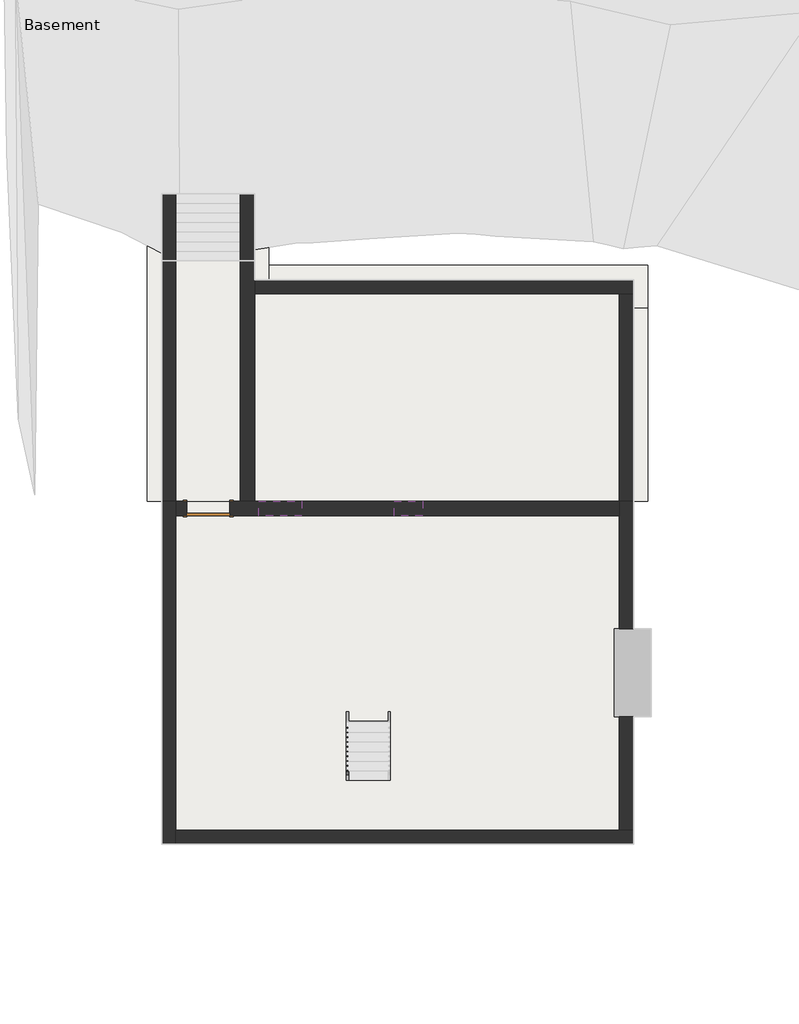
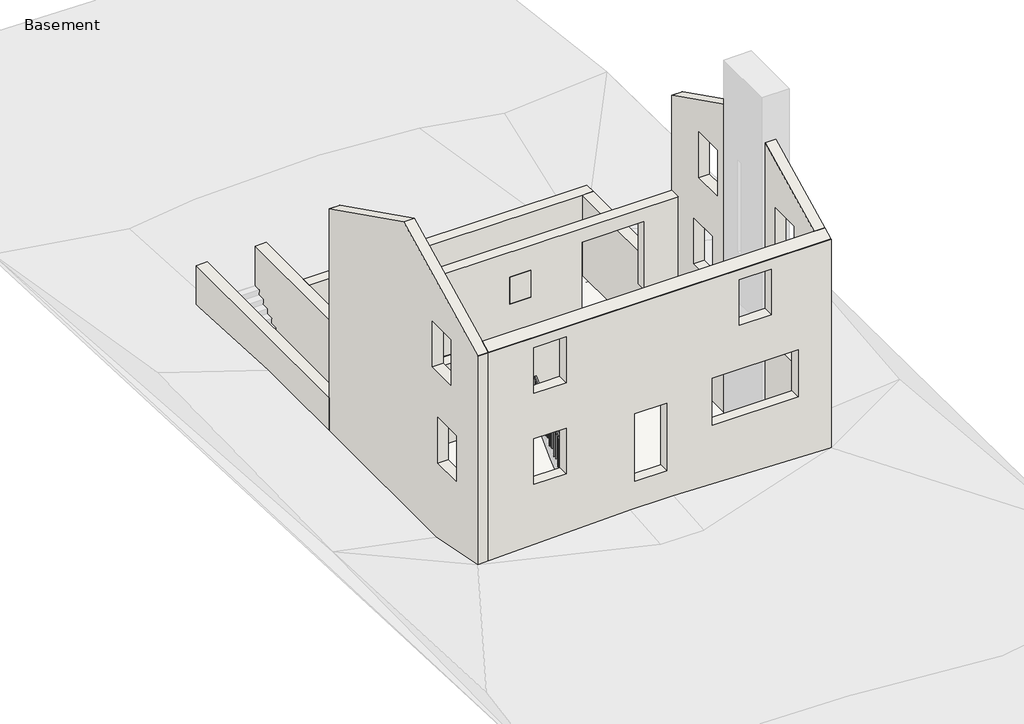
# One storey, part 1 of 2: 11 walls, 4 footings, 4 slabs, 1 door, 1 railing.
"""IFC4 building model written with IfcOpenShell, lengths in millimetres."""

import ifcopenshell
import ifcopenshell.guid

model = None  # the IFC model being written
_history = None  # IfcOwnerHistory: only IFC2X3 demands one
_inside = {}  # id of a spatial element -> (the spatial element, [elements in it])
_under = {}  # id of a project, library or spatial element -> (it, [spatial elements below it])
_declared = {}  # id of a project -> (the project, [libraries it declares])
_typed = {}  # id of a type object -> (the type object, [elements of that type])
_made_of = {}  # id of a material, layer set ... -> (it, [elements and type objects made of it])


def new_model(schema):
    """Start an empty IFC model of exactly this schema.

    Asked for "IFC4X3", IfcOpenShell would pick the latest addendum, in which some entities
    have other attributes; the version numbers below select the first issue.
    IFC2X3 requires an IfcOwnerHistory on every rooted entity: one is made here for all.
    """
    global model, _history
    if schema == "IFC4X3":
        model = ifcopenshell.file(schema_version=(4, 3, 0, 0))
    else:
        model = ifcopenshell.file(schema=schema)
    _inside.clear()
    _under.clear()
    _declared.clear()
    _typed.clear()
    _made_of.clear()
    _history = None
    if model.schema == "IFC2X3":
        org = make("IfcOrganization", Name="unknown")
        user = make(
            "IfcPersonAndOrganization",
            ThePerson=make("IfcPerson", FamilyName="unknown"),
            TheOrganization=org,
        )
        app = make(
            "IfcApplication",
            ApplicationDeveloper=org,
            Version="unknown",
            ApplicationFullName="unknown",
            ApplicationIdentifier="unknown",
        )
        _history = make(
            "IfcOwnerHistory",
            OwningUser=user,
            OwningApplication=app,
            ChangeAction="ADDED",
            CreationDate=0,
        )
    return model


def make(cls, **values):
    """One entity of the class cls with the attributes given. An attribute that is None is left unset."""
    return model.create_entity(
        cls, **{name: value for name, value in values.items() if value is not None}
    )


def rooted(cls, **values):
    """An entity with a GlobalId (a new one), such as an element, a storey or a relation."""
    return make(cls, GlobalId=ifcopenshell.guid.new(), OwnerHistory=_history, **values)


def si_unit(unit_type, name, prefix=None):
    """IfcSIUnit, for example si_unit("LENGTHUNIT", "METRE", prefix="MILLI")."""
    return make("IfcSIUnit", UnitType=unit_type, Prefix=prefix, Name=name)


def assignment(units):
    """IfcUnitAssignment: the units of a project."""
    return None if units is None else make("IfcUnitAssignment", Units=units)


def point(xyz):
    """IfcCartesianPoint."""
    return None if xyz is None else make("IfcCartesianPoint", Coordinates=xyz)


def direction(xyz):
    """IfcDirection."""
    return None if xyz is None else make("IfcDirection", DirectionRatios=xyz)


def frame(location, z_axis=None, x_axis=None):
    """IfcAxis2Placement3D, a coordinate frame: its origin and axes. An axis left out is left unset."""
    return make(
        "IfcAxis2Placement3D",
        Location=point(location),
        Axis=direction(z_axis),
        RefDirection=direction(x_axis),
    )


def origin():
    """The frame at (0, 0, 0) with its axes left unset."""
    return frame((0.0, 0.0, 0.0))


def origin_with_axes():
    """The frame at (0, 0, 0) with the z axis (0, 0, 1) and the x axis (1, 0, 0) written out."""
    return frame((0.0, 0.0, 0.0), z_axis=(0.0, 0.0, 1.0), x_axis=(1.0, 0.0, 0.0))


def place(relative_to, where):
    """IfcLocalPlacement: puts the frame where relative to a parent placement (None: the world)."""
    return make(
        "IfcLocalPlacement", PlacementRelTo=relative_to, RelativePlacement=where
    )


def context(
    kind, dimensions, precision=None, world=None, true_north=None, identifier=None
):
    """IfcGeometricRepresentationContext, for example the 3D "Model" context."""
    return make(
        "IfcGeometricRepresentationContext",
        ContextIdentifier=identifier,
        ContextType=kind,
        CoordinateSpaceDimension=dimensions,
        Precision=precision,
        WorldCoordinateSystem=world,
        TrueNorth=true_north,
    )


def project(units=None, contexts=None):
    """IfcProject with its units and contexts."""
    return rooted(
        "IfcProject",
        Name="project",
        RepresentationContexts=contexts,
        UnitsInContext=assignment(units),
    )


def spatial(cls, under=None, at=None, **own):
    """A site, building, storey or space (cls), placed at a placement, below another one or the project."""
    s = rooted(cls, ObjectPlacement=at, **own)
    if under is not None:
        _under.setdefault(under.id(), (under, []))[1].append(s)
    return s


def polyline(points):
    """IfcPolyline through the points."""
    return make("IfcPolyline", Points=[point(p) for p in points])


def outline(outer, holes=None, kind="AREA"):
    """IfcArbitraryClosedProfileDef: a profile drawn as a closed curve; with holes, ...WithVoids."""
    if holes is None:
        return make("IfcArbitraryClosedProfileDef", ProfileType=kind, OuterCurve=outer)
    return make(
        "IfcArbitraryProfileDefWithVoids",
        ProfileType=kind,
        OuterCurve=outer,
        InnerCurves=holes,
    )


def extrude(swept, where, along, depth):
    """IfcExtrudedAreaSolid: the profile swept, set in the frame where, extruded along a direction by depth."""
    return make(
        "IfcExtrudedAreaSolid",
        SweptArea=swept,
        Position=where,
        ExtrudedDirection=direction(along),
        Depth=depth,
    )


def faces_of(points, faces, orient=None, outer=None):
    """IfcFace entities. A face is a list of loops; a loop is a list of indices into points, from 0.

    orient and outer hold one flag for each loop. By default every Orientation is true, the
    first loop of a face is its IfcFaceOuterBound and the others are IfcFaceBound.
    """
    made = []
    for i, loops in enumerate(faces):
        bounds = []
        for j, loop in enumerate(loops):
            is_outer = j == 0 if outer is None else outer[i][j]
            bounds.append(
                make(
                    "IfcFaceOuterBound" if is_outer else "IfcFaceBound",
                    Bound=make("IfcPolyLoop", Polygon=[points[k] for k in loop]),
                    Orientation=True if orient is None else orient[i][j],
                )
            )
        made.append(make("IfcFace", Bounds=bounds))
    return made


def faceted_brep(points, faces, orient=None, outer=None, voids=None):
    """IfcFacetedBrep: a solid bounded by flat faces; with voids (closed shells), ...WithVoids."""
    shared = [point(p) for p in points]
    hull = make("IfcClosedShell", CfsFaces=faces_of(shared, faces, orient, outer))
    if voids is None:
        return make("IfcFacetedBrep", Outer=hull)
    return make(
        "IfcFacetedBrepWithVoids",
        Outer=hull,
        Voids=[
            make(cls, CfsFaces=faces_of(shared, fs, o, b)) for cls, fs, o, b in voids
        ],
    )


def shape(context_of_items, identifier, shape_type, items):
    """IfcShapeRepresentation: the items that make up one representation, for example the "Body"."""
    return make(
        "IfcShapeRepresentation",
        ContextOfItems=context_of_items,
        RepresentationIdentifier=identifier,
        RepresentationType=shape_type,
        Items=items,
    )


def source(mapping_origin, context_of_items, identifier, shape_type, items):
    """IfcRepresentationMap: a shape defined once, which mapped items show again and again."""
    return make(
        "IfcRepresentationMap",
        MappingOrigin=mapping_origin,
        MappedRepresentation=shape(context_of_items, identifier, shape_type, items),
    )


def transform(
    local_origin,
    x_axis=None,
    y_axis=None,
    z_axis=None,
    scale=None,
    scale2=None,
    scale3=None,
    uniform=True,
):
    """IfcCartesianTransformationOperator3D, or its non-uniform kind. x_axis, y_axis, z_axis: its Axis1, 2, 3."""
    if uniform:
        return make(
            "IfcCartesianTransformationOperator3D",
            Axis1=direction(x_axis),
            Axis2=direction(y_axis),
            LocalOrigin=point(local_origin),
            Scale=scale,
            Axis3=direction(z_axis),
        )
    return make(
        "IfcCartesianTransformationOperator3DnonUniform",
        Axis1=direction(x_axis),
        Axis2=direction(y_axis),
        LocalOrigin=point(local_origin),
        Scale=scale,
        Axis3=direction(z_axis),
        Scale2=scale2,
        Scale3=scale3,
    )


def mapped(mapping_source, mapping_target):
    """IfcMappedItem: shows the shape of a source again, moved by a transform."""
    return make(
        "IfcMappedItem", MappingSource=mapping_source, MappingTarget=mapping_target
    )


def made_of(thing, what):
    """Note that an element or type object is made of a material, layer set ...; save() writes the relation."""
    if what is not None:
        _made_of.setdefault(what.id(), (what, []))[1].append(thing)
    return thing


def element(
    cls,
    number,
    at=None,
    inside=None,
    cuts=None,
    type_object=None,
    material=None,
    context=None,
    identifier="Body",
    shape_type=None,
    held_by="IfcProductDefinitionShape",
    body=None,
    shapes=None,
    **own,
):
    """One element of the class cls, such as IfcWall. Its Tag is "e" and its number.

    at: its placement. inside: the storey or other place that contains it. cuts: it is an
    opening in that element (IfcRelVoidsElement). A single representation is given by context,
    identifier, shape_type and body (its items); several are given by shapes. held_by: the class
    of the entity that holds the representations. save() writes the other relations.
    """
    e = rooted(cls, Tag="e%d" % number, ObjectPlacement=at, **own)
    if body is not None:
        shapes = [shape(context, identifier, shape_type, body)]
    if shapes is not None:
        e.Representation = make(held_by, Representations=shapes)
    if inside is not None:
        _inside.setdefault(inside.id(), (inside, []))[1].append(e)
    if cuts is not None:
        rooted(
            "IfcRelVoidsElement", RelatingBuildingElement=cuts, RelatedOpeningElement=e
        )
    if type_object is not None:
        _typed.setdefault(type_object.id(), (type_object, []))[1].append(e)
    return made_of(e, material)


def aggregate(whole, parts):
    """IfcRelAggregates: a whole, such as a stair, and the parts it consists of."""
    return rooted("IfcRelAggregates", RelatingObject=whole, RelatedObjects=parts)


def save(model, path):
    """Write the relations noted so far, then the file.

    IfcRelAggregates (storeys below a building ...), IfcRelContainedInSpatialStructure (elements
    in a storey), IfcRelDefinesByType, IfcRelAssociatesMaterial and IfcRelDeclares: one each for
    every whole, place, type object, material and project.
    """
    for whole, parts in _under.values():
        aggregate(whole, parts)
    for where, things in _inside.values():
        rooted(
            "IfcRelContainedInSpatialStructure",
            RelatedElements=things,
            RelatingStructure=where,
        )
    for kind, things in _typed.values():
        rooted("IfcRelDefinesByType", RelatedObjects=things, RelatingType=kind)
    for what, things in _made_of.values():
        rooted("IfcRelAssociatesMaterial", RelatedObjects=things, RelatingMaterial=what)
    for by, libraries in _declared.values():
        rooted("IfcRelDeclares", RelatingContext=by, RelatedDefinitions=libraries)
    model.write(path)


def door_03272193(model_context):
    return source(origin(), model_context, "Body", "SweptSolid", [
        extrude(outline(polyline([(2209.8, -533.4), (0.0, -533.4), (0.0, -457.2), (2133.6, -457.2), (2133.6, 457.2), (0.0, 457.2), (0.0, 533.4), (2209.8, 533.4), (2209.8, -533.4)])), frame((0.0, 152.4, 0.0), z_axis=(0.0, 1.0, 0.0), x_axis=(0.0, 0.0, 1.0)), (0.0, 0.0, 1.0), 25.4),
        extrude(outline(polyline([(2209.8, 533.4), (2209.8, -533.4), (0.0, -533.4), (0.0, -457.2), (2133.6, -457.2), (2133.6, 457.2), (0.0, 457.2), (0.0, 533.4), (2209.8, 533.4)])), frame((0.0, -177.8, 0.0), z_axis=(0.0, 1.0, 0.0), x_axis=(0.0, 0.0, 1.0)), (0.0, 0.0, 1.0), 25.4),
        extrude(outline(polyline([(457.2, 101.6), (-457.2, 101.6), (-457.2, 152.4), (457.2, 152.4), (457.2, 101.6)])), origin_with_axes(), (0.0, 0.0, 1.0), 2133.6),
    ])


model = new_model("IFC4")

# Units and contexts
model_context = context("Model", 3, world=origin())
ifc_project = project(units=[si_unit("LENGTHUNIT", "METRE", prefix="MILLI")], contexts=[model_context])

# Site, building, storey
site = spatial("IfcSite", under=ifc_project)
building = spatial("IfcBuilding", under=site)
storey = spatial("IfcBuildingStorey", under=building, Name="Basement", Elevation=-2667.0)

# Door
placement = place(None, origin())
door_shape = door_03272193(model_context)
element("IfcDoor", 1, ObjectType="Single-Flush : 36\" x 84\"", at=placement, inside=storey, context=model_context, shape_type="MappedRepresentation", body=[
    mapped(door_shape, transform((-4998.5803068, 2999.6888758, -2667.0), x_axis=(-1.0, 0.0, 0.0), y_axis=(0.0, -1.0, 0.0), z_axis=(0.0, 0.0, 1.0))),
])

# Footings
element("IfcFooting", 2, ObjectType="Bearing Footing - 36\" x 12\"", at=placement, inside=storey, context=model_context, shape_type="SweptSolid", body=[
    extrude(outline(polyline([(-5379.5803068, 3152.0888758), (-6293.9803068, 3152.0888758), (-6293.9803068, 10010.0888758), (-5379.5803068, 10010.0888758), (-5379.5803068, 3152.0888758)])), frame((0.0, 0.0, -3073.4), z_axis=(0.0, 0.0, 1.0), x_axis=(1.0, 0.0, 0.0)), (0.0, 0.0, 1.0), 304.8),
])
element("IfcFooting", 3, ObjectType="Bearing Footing - 36\" x 12\"", at=placement, inside=storey, context=model_context, shape_type="Brep", body=[
    faceted_brep([(-3703.1803068, 7266.8888758, -2768.6), (3459.6196932, 7266.8888758, -2768.6), (4374.0196932, 7266.8888758, -2768.6), (4374.0196932, 8181.2888758, -2768.6), (-3703.1803068, 8181.2888758, -2768.6), (-3703.1803068, 8181.2888758, -3073.4), (4374.0196932, 8181.2888758, -3073.4), (-3703.1803068, 7266.8888758, -3073.4), (4374.0196932, 7266.8888758, -3073.4), (3459.6196932, 7266.8888758, -3073.4)], [[[0, 1, 2, 3, 4]], [[5, 4, 3, 6]], [[7, 5, 6, 8, 9]], [[0, 7, 9, 8, 2, 1]], [[0, 4, 5, 7]], [[3, 2, 8, 6]]]),
])
element("IfcFooting", 4, ObjectType="Bearing Footing - 36\" x 12\"", at=placement, inside=storey, context=model_context, shape_type="SweptSolid", body=[
    extrude(outline(polyline([(4374.0196932, 3152.0888758), (3459.6196932, 3152.0888758), (3459.6196932, 7266.8888758), (4374.0196932, 7266.8888758), (4374.0196932, 3152.0888758)])), frame((0.0, 0.0, -3073.4), z_axis=(0.0, 0.0, 1.0), x_axis=(1.0, 0.0, 0.0)), (0.0, 0.0, 1.0), 304.8),
])
element("IfcFooting", 5, ObjectType="Bearing Footing - 36\" x 12\"", at=placement, inside=storey, context=model_context, shape_type="Brep", body=[
    faceted_brep([(-3703.1803068, 3152.0888758, -2768.6), (-4617.5803068, 3152.0888758, -2768.6), (-4617.5803068, 3152.0888758, -3073.4), (-3703.1803068, 3152.0888758, -3073.4), (-4617.5803068, 10010.0888758, -2768.6), (-3703.1803068, 10010.0888758, -2768.6), (-3703.1803068, 10010.0888758, -3073.4), (-4617.5803068, 10010.0888758, -3073.4), (-3703.1803068, 7266.8888758, -2768.6), (-3703.1803068, 8181.2888758, -2768.6), (-3703.1803068, 8181.2888758, -3073.4), (-3703.1803068, 7266.8888758, -3073.4)], [[[0, 1, 2, 3]], [[4, 5, 6, 7]], [[0, 8, 9, 5, 4, 1]], [[2, 1, 4, 7]], [[3, 2, 7, 6, 10, 11]], [[0, 3, 11, 10, 6, 5, 9, 8]]]),
])

# Railing
element("IfcRailing", 6, ObjectType="Handrail - Rectangular", at=placement, inside=storey, context=model_context, shape_type="SweptSolid", body=[
    extrude(outline(polyline([(-2791.5111242, -1631.7331862), (-2791.5111242, -1562.1), (-149.9111242, 914.4), (-149.9111242, 844.7668138), (-2791.5111242, -1631.7331862)])), frame((-2052.1803068, 0.0, 0.0), z_axis=(1.0, 0.0, 0.0), x_axis=(0.0, 1.0, 0.0)), (0.0, 0.0, 1.0), 50.8),
    extrude(outline(polyline([(-241.9861242, 758.4465013), (-241.9861242, -190.5), (-261.0361242, -190.5), (-261.0361242, 740.5871263), (-241.9861242, 758.4465013)])), frame((-2036.3053068, 0.0, 0.0), z_axis=(1.0, 0.0, 0.0), x_axis=(0.0, 1.0, 0.0)), (0.0, 0.0, 1.0), 19.05),
    extrude(outline(polyline([(-343.5861242, 663.1965013), (-343.5861242, -190.5), (-362.6361242, -190.5), (-362.6361242, 645.3371263), (-343.5861242, 663.1965013)])), frame((-2036.3053068, 0.0, 0.0), z_axis=(1.0, 0.0, 0.0), x_axis=(0.0, 1.0, 0.0)), (0.0, 0.0, 1.0), 19.05),
    extrude(outline(polyline([(-445.1861242, 567.9465013), (-445.1861242, -381.0), (-464.2361242, -381.0), (-464.2361242, 550.0871263), (-445.1861242, 567.9465013)])), frame((-2036.3053068, 0.0, 0.0), z_axis=(1.0, 0.0, 0.0), x_axis=(0.0, 1.0, 0.0)), (0.0, 0.0, 1.0), 19.05),
    extrude(outline(polyline([(-546.7861242, 472.6965013), (-546.7861242, -381.0), (-565.8361242, -381.0), (-565.8361242, 454.8371263), (-546.7861242, 472.6965013)])), frame((-2036.3053068, 0.0, 0.0), z_axis=(1.0, 0.0, 0.0), x_axis=(0.0, 1.0, 0.0)), (0.0, 0.0, 1.0), 19.05),
    extrude(outline(polyline([(-648.3861242, 377.4465013), (-648.3861242, -571.5), (-667.4361242, -571.5), (-667.4361242, 359.5871263), (-648.3861242, 377.4465013)])), frame((-2036.3053068, 0.0, 0.0), z_axis=(1.0, 0.0, 0.0), x_axis=(0.0, 1.0, 0.0)), (0.0, 0.0, 1.0), 19.05),
    extrude(outline(polyline([(-749.9861242, 282.1965013), (-749.9861242, -571.5), (-769.0361242, -571.5), (-769.0361242, 264.3371263), (-749.9861242, 282.1965013)])), frame((-2036.3053068, 0.0, 0.0), z_axis=(1.0, 0.0, 0.0), x_axis=(0.0, 1.0, 0.0)), (0.0, 0.0, 1.0), 19.05),
    extrude(outline(polyline([(-851.5861242, 186.9465013), (-851.5861242, -762.0), (-870.6361242, -762.0), (-870.6361242, 169.0871263), (-851.5861242, 186.9465013)])), frame((-2036.3053068, 0.0, 0.0), z_axis=(1.0, 0.0, 0.0), x_axis=(0.0, 1.0, 0.0)), (0.0, 0.0, 1.0), 19.05),
    extrude(outline(polyline([(-953.1861242, 91.6965013), (-953.1861242, -762.0), (-972.2361242, -762.0), (-972.2361242, 73.8371263), (-953.1861242, 91.6965013)])), frame((-2036.3053068, 0.0, 0.0), z_axis=(1.0, 0.0, 0.0), x_axis=(0.0, 1.0, 0.0)), (0.0, 0.0, 1.0), 19.05),
    extrude(outline(polyline([(-1054.7861242, -3.5534987), (-1054.7861242, -952.5), (-1073.8361242, -952.5), (-1073.8361242, -21.4128737), (-1054.7861242, -3.5534987)])), frame((-2036.3053068, 0.0, 0.0), z_axis=(1.0, 0.0, 0.0), x_axis=(0.0, 1.0, 0.0)), (0.0, 0.0, 1.0), 19.05),
    extrude(outline(polyline([(-1156.3861242, -98.8034987), (-1156.3861242, -952.5), (-1175.4361242, -952.5), (-1175.4361242, -116.6628737), (-1156.3861242, -98.8034987)])), frame((-2036.3053068, 0.0, 0.0), z_axis=(1.0, 0.0, 0.0), x_axis=(0.0, 1.0, 0.0)), (0.0, 0.0, 1.0), 19.05),
    extrude(outline(polyline([(-1257.9861242, -194.0534987), (-1257.9861242, -1143.0), (-1277.0361242, -1143.0), (-1277.0361242, -211.9128737), (-1257.9861242, -194.0534987)])), frame((-2036.3053068, 0.0, 0.0), z_axis=(1.0, 0.0, 0.0), x_axis=(0.0, 1.0, 0.0)), (0.0, 0.0, 1.0), 19.05),
    extrude(outline(polyline([(-1359.5861242, -289.3034987), (-1359.5861242, -1143.0), (-1378.6361242, -1143.0), (-1378.6361242, -307.1628737), (-1359.5861242, -289.3034987)])), frame((-2036.3053068, 0.0, 0.0), z_axis=(1.0, 0.0, 0.0), x_axis=(0.0, 1.0, 0.0)), (0.0, 0.0, 1.0), 19.05),
    extrude(outline(polyline([(-1461.1861242, -384.5534987), (-1461.1861242, -1333.5), (-1480.2361242, -1333.5), (-1480.2361242, -402.4128737), (-1461.1861242, -384.5534987)])), frame((-2036.3053068, 0.0, 0.0), z_axis=(1.0, 0.0, 0.0), x_axis=(0.0, 1.0, 0.0)), (0.0, 0.0, 1.0), 19.05),
    extrude(outline(polyline([(-1562.7861242, -479.8034987), (-1562.7861242, -1333.5), (-1581.8361242, -1333.5), (-1581.8361242, -497.6628737), (-1562.7861242, -479.8034987)])), frame((-2036.3053068, 0.0, 0.0), z_axis=(1.0, 0.0, 0.0), x_axis=(0.0, 1.0, 0.0)), (0.0, 0.0, 1.0), 19.05),
    extrude(outline(polyline([(-1664.3861242, -575.0534987), (-1664.3861242, -1524.0), (-1683.4361242, -1524.0), (-1683.4361242, -592.9128737), (-1664.3861242, -575.0534987)])), frame((-2036.3053068, 0.0, 0.0), z_axis=(1.0, 0.0, 0.0), x_axis=(0.0, 1.0, 0.0)), (0.0, 0.0, 1.0), 19.05),
    extrude(outline(polyline([(-1765.9861242, -670.3034987), (-1765.9861242, -1524.0), (-1785.0361242, -1524.0), (-1785.0361242, -688.1628737), (-1765.9861242, -670.3034987)])), frame((-2036.3053068, 0.0, 0.0), z_axis=(1.0, 0.0, 0.0), x_axis=(0.0, 1.0, 0.0)), (0.0, 0.0, 1.0), 19.05),
    extrude(outline(polyline([(-1867.5861242, -765.5534987), (-1867.5861242, -1714.5), (-1886.6361242, -1714.5), (-1886.6361242, -783.4128737), (-1867.5861242, -765.5534987)])), frame((-2036.3053068, 0.0, 0.0), z_axis=(1.0, 0.0, 0.0), x_axis=(0.0, 1.0, 0.0)), (0.0, 0.0, 1.0), 19.05),
    extrude(outline(polyline([(-1969.1861242, -860.8034987), (-1969.1861242, -1714.5), (-1988.2361242, -1714.5), (-1988.2361242, -878.6628737), (-1969.1861242, -860.8034987)])), frame((-2036.3053068, 0.0, 0.0), z_axis=(1.0, 0.0, 0.0), x_axis=(0.0, 1.0, 0.0)), (0.0, 0.0, 1.0), 19.05),
    extrude(outline(polyline([(-2070.7861242, -956.0534987), (-2070.7861242, -1905.0), (-2089.8361242, -1905.0), (-2089.8361242, -973.9128737), (-2070.7861242, -956.0534987)])), frame((-2036.3053068, 0.0, 0.0), z_axis=(1.0, 0.0, 0.0), x_axis=(0.0, 1.0, 0.0)), (0.0, 0.0, 1.0), 19.05),
    extrude(outline(polyline([(-2172.3861242, -1051.3034987), (-2172.3861242, -1905.0), (-2191.4361242, -1905.0), (-2191.4361242, -1069.1628737), (-2172.3861242, -1051.3034987)])), frame((-2036.3053068, 0.0, 0.0), z_axis=(1.0, 0.0, 0.0), x_axis=(0.0, 1.0, 0.0)), (0.0, 0.0, 1.0), 19.05),
    extrude(outline(polyline([(-2273.9861242, -1146.5534987), (-2273.9861242, -2095.5), (-2293.0361242, -2095.5), (-2293.0361242, -1164.4128737), (-2273.9861242, -1146.5534987)])), frame((-2036.3053068, 0.0, 0.0), z_axis=(1.0, 0.0, 0.0), x_axis=(0.0, 1.0, 0.0)), (0.0, 0.0, 1.0), 19.05),
    extrude(outline(polyline([(-2375.5861242, -1241.8034987), (-2375.5861242, -2095.5), (-2394.6361242, -2095.5), (-2394.6361242, -1259.6628737), (-2375.5861242, -1241.8034987)])), frame((-2036.3053068, 0.0, 0.0), z_axis=(1.0, 0.0, 0.0), x_axis=(0.0, 1.0, 0.0)), (0.0, 0.0, 1.0), 19.05),
    extrude(outline(polyline([(-2477.1861242, -1337.0534987), (-2477.1861242, -2286.0), (-2496.2361242, -2286.0), (-2496.2361242, -1354.9128737), (-2477.1861242, -1337.0534987)])), frame((-2036.3053068, 0.0, 0.0), z_axis=(1.0, 0.0, 0.0), x_axis=(0.0, 1.0, 0.0)), (0.0, 0.0, 1.0), 19.05),
    extrude(outline(polyline([(-2578.7861242, -1432.3034987), (-2578.7861242, -2286.0), (-2597.8361242, -2286.0), (-2597.8361242, -1450.1628737), (-2578.7861242, -1432.3034987)])), frame((-2036.3053068, 0.0, 0.0), z_axis=(1.0, 0.0, 0.0), x_axis=(0.0, 1.0, 0.0)), (0.0, 0.0, 1.0), 19.05),
    extrude(outline(polyline([(-2680.3861242, -1527.5534987), (-2680.3861242, -2476.5), (-2699.4361242, -2476.5), (-2699.4361242, -1545.4128737), (-2680.3861242, -1527.5534987)])), frame((-2036.3053068, 0.0, 0.0), z_axis=(1.0, 0.0, 0.0), x_axis=(0.0, 1.0, 0.0)), (0.0, 0.0, 1.0), 19.05),
    extrude(outline(polyline([(-149.9111242, 844.7668138), (-149.9111242, -190.5), (-168.9611242, -190.5), (-168.9611242, 826.9074388), (-149.9111242, 844.7668138)])), frame((-2036.3053068, 0.0, 0.0), z_axis=(1.0, 0.0, 0.0), x_axis=(0.0, 1.0, 0.0)), (0.0, 0.0, 1.0), 19.05),
    extrude(outline(polyline([(-2772.4611242, -1613.8738112), (-2772.4611242, -2476.5), (-2791.5111242, -2476.5), (-2791.5111242, -1631.7331862), (-2772.4611242, -1613.8738112)])), frame((-2036.3053068, 0.0, 0.0), z_axis=(1.0, 0.0, 0.0), x_axis=(0.0, 1.0, 0.0)), (0.0, 0.0, 1.0), 19.05),
])

# Slabs
element("IfcSlab", 7, ObjectType="4\" Concrete", at=placement, inside=storey, context=model_context, shape_type="SweptSolid", body=[
    extrude(outline(polyline([(-5684.3803068, 8384.4888758), (-4312.7803068, 8384.4888758), (-4312.7803068, 3152.0888758), (-5684.3803068, 3152.0888758), (-5684.3803068, 8384.4888758)])), frame((0.0, 0.0, -2768.6), z_axis=(0.0, 0.0, 1.0), x_axis=(1.0, 0.0, 0.0)), (0.0, 0.0, 1.0), 101.6),
])
element("IfcSlab", 8, ObjectType="Pad 1", at=placement, inside=storey, context=model_context, shape_type="SweptSolid", body=[
    extrude(outline(polyline([(4069.2196932, 434.2888758), (4450.2196932, 434.2888758), (4450.2196932, -1445.3111242), (4069.2196932, -1445.3111242), (4069.2196932, -4163.1111242), (-5989.1803068, -4163.1111242), (-5989.1803068, 3152.0888758), (4069.2196932, 3152.0888758), (4069.2196932, 434.2888758)])), frame((0.0, 0.0, -3073.4), z_axis=(0.0, 0.0, 1.0), x_axis=(1.0, 0.0, 0.0)), (0.0, 0.0, 1.0), 304.8),
])
element("IfcSlab", 9, ObjectType="Pad 1", at=placement, inside=storey, context=model_context, shape_type="SweptSolid", body=[
    extrude(outline(polyline([(-5989.1803068, 8275.4102719), (-4007.9803068, 8275.4102719), (-4007.9803068, 7876.4888758), (4069.2196932, 7876.4888758), (4069.2196932, 3152.0888758), (-5989.1803068, 3152.0888758), (-5989.1803068, 8275.4102719)])), frame((0.0, 0.0, -3073.4), z_axis=(0.0, 0.0, 1.0), x_axis=(1.0, 0.0, 0.0)), (0.0, 0.0, 1.0), 304.8),
])
element("IfcSlab", 10, ObjectType="Under Stairs", at=placement, inside=storey, context=model_context, shape_type="SweptSolid", body=[
    extrude(outline(polyline([(9705.2888758, -1653.200634), (8275.4102719, -2776.6756068), (8275.4102719, -2768.6), (9705.2888758, -1645.1250272), (9705.2888758, -1653.200634)])), frame((-5989.1803068, 0.0, 0.0), z_axis=(1.0, 0.0, 0.0), x_axis=(0.0, 1.0, 0.0)), (0.0, 0.0, 1.0), 1981.2),
])

# Walls
element("IfcWall", 11, ObjectType="Foundation - 12\" Concrete", at=placement, inside=storey, context=model_context, shape_type="Brep", body=[
    faceted_brep([(-5684.3803068, 3152.0888758, -2768.6), (-5684.3803068, 8384.4888758, -2768.6), (-5684.3803068, 9705.2888758, -2768.6), (-5684.3803068, 9705.2888758, -349.25), (-5684.3803068, 3152.0888758, -349.25), (-5684.3803068, 3152.0888758, -2667.0), (-5989.1803068, 3152.0888758, -2768.6), (-5989.1803068, 3152.0888758, -349.25), (-5989.1803068, 9705.2888758, -349.25), (-5989.1803068, 9705.2888758, -2768.6)], [[[0, 1, 2, 3, 4, 5]], [[6, 7, 8, 9]], [[2, 1, 0, 6, 9]], [[3, 2, 9, 8]], [[4, 3, 8, 7]], [[0, 5, 4, 7, 6]]]),
])
element("IfcWall", 12, ObjectType="Foundation - 12\" Concrete", at=placement, inside=storey, context=model_context, shape_type="Brep", body=[
    faceted_brep([(-4007.9803068, 7571.6888758, -2768.6), (3764.4196932, 7571.6888758, -2768.6), (4069.2196932, 7571.6888758, -2768.6), (4069.2196932, 7571.6888758, -349.25), (3764.4196932, 7571.6888758, -349.25), (-4007.9803068, 7571.6888758, -349.25), (-4007.9803068, 7876.4888758, -2768.6), (-4007.9803068, 7876.4888758, -349.25), (4069.2196932, 7876.4888758, -349.25), (4069.2196932, 7876.4888758, -2768.6)], [[[0, 1, 2, 3, 4, 5]], [[6, 7, 8, 9]], [[2, 1, 0, 6, 9]], [[5, 4, 3, 8, 7]], [[3, 2, 9, 8]], [[0, 5, 7, 6]]]),
])
element("IfcWall", 13, ObjectType="Foundation - 12\" Concrete", at=placement, inside=storey, context=model_context, shape_type="Brep", body=[
    faceted_brep([(3764.4196932, 7571.6888758, -2768.6), (3764.4196932, 3152.0888758, -2768.6), (3764.4196932, 3152.0888758, -349.25), (3764.4196932, 7571.6888758, -349.25), (4069.2196932, 7571.6888758, -2768.6), (4069.2196932, 7571.6888758, -349.25), (4069.2196932, 7524.0638758, -349.25), (4069.2196932, 3152.0888758, -349.25), (4069.2196932, 3152.0888758, -2768.6)], [[[0, 1, 2, 3]], [[4, 5, 6, 7, 8]], [[1, 0, 4, 8]], [[3, 2, 7, 6, 5]], [[2, 1, 8, 7]], [[0, 3, 5, 4]]]),
])
element("IfcWall", 14, ObjectType="Foundation - 12\" Concrete", at=placement, inside=storey, context=model_context, shape_type="Brep", body=[
    faceted_brep([(-4007.9803068, 3152.0888758, -2768.6), (-4007.9803068, 7571.6888758, -2768.6), (-4007.9803068, 7876.4888758, -2768.6), (-4007.9803068, 9705.2888758, -2768.6), (-4007.9803068, 9705.2888758, -349.25), (-4007.9803068, 7876.4888758, -349.25), (-4007.9803068, 7571.6888758, -349.25), (-4007.9803068, 3152.0888758, -349.25), (-4312.7803068, 3152.0888758, -2768.6), (-4312.7803068, 3152.0888758, -2667.0), (-4312.7803068, 3152.0888758, -349.25), (-4312.7803068, 9705.2888758, -349.25), (-4312.7803068, 9705.2888758, -2768.6), (-4312.7803068, 8384.4888758, -2768.6)], [[[0, 1, 2, 3, 4, 5, 6, 7]], [[8, 9, 10, 11, 12, 13]], [[3, 2, 1, 0, 8, 13, 12]], [[4, 3, 12, 11]], [[7, 6, 5, 4, 11, 10]], [[0, 7, 10, 9, 8]]]),
])
element("IfcWall", 15, ObjectType="Generic - 12\"", at=placement, inside=storey, context=model_context, shape_type="Brep", body=[
    faceted_brep([(1021.2196932, 2847.2888758, 0.0), (1021.2196932, 2847.2888758, 2057.4), (2799.2196932, 2847.2888758, 2057.4), (2799.2196932, 2847.2888758, 0.0), (3764.4196932, 2847.2888758, 0.0), (3764.4196932, 2847.2888758, 2470.15), (-5684.3803068, 2847.2888758, 2470.15), (-5684.3803068, 2847.2888758, 0.0), (-5023.9803068, 2847.2888758, 0.0), (-5023.9803068, 2847.2888758, 2032.0), (-4160.3803068, 2847.2888758, 2032.0), (-4160.3803068, 2847.2888758, 0.0), (-1518.7803068, 2847.2888758, 0.0), (-1391.7803068, 2847.2888758, 0.0), (-70.9803068, 2847.2888758, 0.0), (56.0196932, 2847.2888758, 0.0), (-3919.0803068, 2847.2888758, 914.4), (-3919.0803068, 2847.2888758, 1727.2), (-3004.6803068, 2847.2888758, 1727.2), (-3004.6803068, 2847.2888758, 914.4), (-1036.1803068, 2847.2888758, 914.4), (-1036.1803068, 2847.2888758, 1727.2), (-426.5803068, 2847.2888758, 1727.2), (-426.5803068, 2847.2888758, 914.4), (1021.2196932, 3152.0888758, 2057.4), (1021.2196932, 3152.0888758, 0.0), (-4160.3803068, 3152.0888758, 0.0), (-4160.3803068, 3152.0888758, 2032.0), (-5023.9803068, 3152.0888758, 2032.0), (-5023.9803068, 3152.0888758, 0.0), (-5684.3803068, 3152.0888758, 0.0), (-5684.3803068, 3152.0888758, 2470.15), (3764.4196932, 3152.0888758, 2470.15), (3764.4196932, 3152.0888758, 0.0), (2799.2196932, 3152.0888758, 0.0), (2799.2196932, 3152.0888758, 2057.4), (-3919.0803068, 3152.0888758, 1727.2), (-3919.0803068, 3152.0888758, 914.4), (-3004.6803068, 3152.0888758, 914.4), (-3004.6803068, 3152.0888758, 1727.2), (-1036.1803068, 3152.0888758, 1727.2), (-1036.1803068, 3152.0888758, 914.4), (-426.5803068, 3152.0888758, 914.4), (-426.5803068, 3152.0888758, 1727.2)], [[[0, 1, 2, 3, 4, 5, 6, 7, 8, 9, 10, 11, 12, 13, 14, 15], [16, 17, 18, 19], [20, 21, 22, 23]], [[24, 25, 26, 27, 28, 29, 30, 31, 32, 33, 34, 35], [36, 37, 38, 39], [40, 41, 42, 43]], [[24, 1, 0, 25]], [[1, 24, 35, 2]], [[2, 35, 34, 3]], [[9, 8, 29, 28]], [[10, 9, 28, 27]], [[11, 10, 27, 26]], [[8, 7, 30, 29]], [[4, 3, 34, 33]], [[0, 15, 14, 13, 12, 11, 26, 25]], [[6, 5, 32, 31]], [[4, 33, 32, 5]], [[36, 17, 16, 37]], [[37, 16, 19, 38]], [[38, 19, 18, 39]], [[17, 36, 39, 18]], [[40, 21, 20, 41]], [[41, 20, 23, 42]], [[42, 23, 22, 43]], [[21, 40, 43, 22]], [[30, 7, 6, 31]]]),
    faceted_brep([(3764.4196932, 2847.2888758, -273.05), (-5684.3803068, 2847.2888758, -273.05), (-5684.3803068, 2847.2888758, -2667.0), (-5455.7803068, 2847.2888758, -2667.0), (-5455.7803068, 2847.2888758, -533.4), (-4541.3803068, 2847.2888758, -533.4), (-4541.3803068, 2847.2888758, -2667.0), (3764.4196932, 2847.2888758, -2667.0), (-5684.3803068, 3152.0888758, -273.05), (3764.4196932, 3152.0888758, -273.05), (3764.4196932, 3152.0888758, -2667.0), (-4541.3803068, 3152.0888758, -2667.0), (-4541.3803068, 3152.0888758, -533.4), (-5455.7803068, 3152.0888758, -533.4), (-5455.7803068, 3152.0888758, -2667.0), (-5684.3803068, 3152.0888758, -2667.0)], [[[0, 1, 2, 3, 4, 5, 6, 7]], [[8, 9, 10, 11, 12, 13, 14, 15]], [[10, 7, 6, 11]], [[3, 2, 15, 14]], [[1, 0, 9, 8]], [[7, 10, 9, 0]], [[13, 4, 3, 14]], [[4, 13, 12, 5]], [[5, 12, 11, 6]], [[15, 2, 1, 8]]]),
])
element("IfcWall", 16, ObjectType="Generic - 12\"", at=placement, inside=storey, context=model_context, shape_type="Brep", body=[
    faceted_brep([(-5684.3803068, -4163.1111242, -2667.0), (-5684.3803068, -3858.3111242, -2667.0), (-5684.3803068, 2847.2888758, -2667.0), (-5684.3803068, 3152.0888758, -2667.0), (-5684.3803068, 3152.0888758, -273.05), (-5684.3803068, 3152.0888758, 0.0), (-5684.3803068, 3152.0888758, 2470.15), (-5684.3803068, 3152.0888758, 5336.1342644), (-5684.3803068, 3147.820347, 5336.1342644), (-5684.3803068, -505.5111242, 7162.8), (-5684.3803068, -3858.3111242, 5486.4), (-5684.3803068, -4158.8425953, 5336.1342644), (-5684.3803068, -4163.1111242, 5336.1342644), (-5684.3803068, -3096.3111242, 914.4), (-5684.3803068, -3096.3111242, 2286.0), (-5684.3803068, -2181.9111242, 2286.0), (-5684.3803068, -2181.9111242, 914.4), (-5684.3803068, -2842.3111242, 3657.6), (-5684.3803068, -2842.3111242, 5029.2), (-5684.3803068, -1927.9111242, 5029.2), (-5684.3803068, -1927.9111242, 3657.6), (-5989.1803068, 3152.0888758, -2667.0), (-5989.1803068, -4163.1111242, -2667.0), (-5989.1803068, -4163.1111242, 5336.1342644), (-5989.1803068, -4158.8425953, 5336.1342644), (-5989.1803068, -505.5111242, 7162.8), (-5989.1803068, 3147.820347, 5336.1342644), (-5989.1803068, 3152.0888758, 5336.1342644), (-5989.1803068, -3096.3111242, 2286.0), (-5989.1803068, -3096.3111242, 914.4), (-5989.1803068, -2181.9111242, 914.4), (-5989.1803068, -2181.9111242, 2286.0), (-5989.1803068, -2842.3111242, 5029.2), (-5989.1803068, -2842.3111242, 3657.6), (-5989.1803068, -1927.9111242, 3657.6), (-5989.1803068, -1927.9111242, 5029.2)], [[[0, 1, 2, 3, 4, 5, 6, 7, 8, 9, 10, 11, 12], [13, 14, 15, 16], [17, 18, 19, 20]], [[21, 22, 23, 24, 25, 26, 27], [28, 29, 30, 31], [32, 33, 34, 35]], [[3, 2, 1, 0, 22, 21]], [[0, 12, 23, 22]], [[29, 28, 14, 13]], [[30, 29, 13, 16]], [[31, 30, 16, 15]], [[28, 31, 15, 14]], [[32, 18, 17, 33]], [[33, 17, 20, 34]], [[34, 20, 19, 35]], [[18, 32, 35, 19]], [[23, 12, 11, 24]], [[25, 24, 11, 10, 9]], [[9, 8, 26, 25]], [[8, 7, 27, 26]], [[3, 21, 27, 7, 6, 5, 4]]]),
])
element("IfcWall", 17, ObjectType="Generic - 12\"", at=placement, inside=storey, context=model_context, shape_type="Brep", body=[
    faceted_brep([(4069.2196932, -3858.3111242, -2667.0), (3764.4196932, -3858.3111242, -2667.0), (-5684.3803068, -3858.3111242, -2667.0), (-5684.3803068, -3858.3111242, 5486.4), (3764.4196932, -3858.3111242, 5486.4), (4069.2196932, -3858.3111242, 5486.4), (-1518.7803068, -3858.3111242, 0.0), (-604.3803068, -3858.3111242, 0.0), (-604.3803068, -3858.3111242, 2032.0), (-1518.7803068, -3858.3111242, 2032.0), (-3474.5803068, -3858.3111242, 914.4), (-3474.5803068, -3858.3111242, 2286.0), (-4388.9803068, -3858.3111242, 2286.0), (-4388.9803068, -3858.3111242, 914.4), (2367.4196932, -3858.3111242, 3657.6), (2367.4196932, -3858.3111242, 5029.2), (1453.0196932, -3858.3111242, 5029.2), (1453.0196932, -3858.3111242, 3657.6), (-3474.5803068, -3858.3111242, 3657.6), (-3474.5803068, -3858.3111242, 5029.2), (-4388.9803068, -3858.3111242, 5029.2), (-4388.9803068, -3858.3111242, 3657.6), (3129.4196932, -3858.3111242, 2336.8), (691.0196932, -3858.3111242, 2336.8), (691.0196932, -3858.3111242, 914.4), (3129.4196932, -3858.3111242, 914.4), (-5684.3803068, -4163.1111242, -2667.0), (4069.2196932, -4163.1111242, -2667.0), (4069.2196932, -4163.1111242, 5336.1342644), (-5684.3803068, -4163.1111242, 5336.1342644), (-604.3803068, -4163.1111242, 0.0), (-1518.7803068, -4163.1111242, 0.0), (-1518.7803068, -4163.1111242, 2032.0), (-604.3803068, -4163.1111242, 2032.0), (-3474.5803068, -4163.1111242, 2286.0), (-3474.5803068, -4163.1111242, 914.4), (-4388.9803068, -4163.1111242, 914.4), (-4388.9803068, -4163.1111242, 2286.0), (2367.4196932, -4163.1111242, 5029.2), (2367.4196932, -4163.1111242, 3657.6), (1453.0196932, -4163.1111242, 3657.6), (1453.0196932, -4163.1111242, 5029.2), (-3474.5803068, -4163.1111242, 5029.2), (-3474.5803068, -4163.1111242, 3657.6), (-4388.9803068, -4163.1111242, 3657.6), (-4388.9803068, -4163.1111242, 5029.2), (3129.4196932, -4163.1111242, 914.4), (691.0196932, -4163.1111242, 914.4), (691.0196932, -4163.1111242, 2336.8), (3129.4196932, -4163.1111242, 2336.8), (4069.2196932, -4158.8425953, 5336.1342644), (-5684.3803068, -4158.8425953, 5336.1342644)], [[[0, 1, 2, 3, 4, 5], [6, 7, 8, 9], [10, 11, 12, 13], [14, 15, 16, 17], [18, 19, 20, 21], [22, 23, 24, 25]], [[26, 27, 28, 29], [30, 31, 32, 33], [34, 35, 36, 37], [38, 39, 40, 41], [42, 43, 44, 45], [46, 47, 48, 49]], [[2, 1, 0, 27, 26]], [[0, 5, 50, 28, 27]], [[3, 2, 26, 29, 51]], [[31, 30, 7, 6]], [[32, 31, 6, 9]], [[33, 32, 9, 8]], [[30, 33, 8, 7]], [[35, 34, 11, 10]], [[36, 35, 10, 13]], [[37, 36, 13, 12]], [[34, 37, 12, 11]], [[24, 47, 46, 25]], [[48, 23, 22, 49]], [[23, 48, 47, 24]], [[25, 46, 49, 22]], [[15, 14, 39, 38]], [[14, 17, 40, 39]], [[17, 16, 41, 40]], [[16, 15, 38, 41]], [[19, 18, 43, 42]], [[18, 21, 44, 43]], [[21, 20, 45, 44]], [[20, 19, 42, 45]], [[5, 4, 3, 51, 50]], [[29, 28, 50, 51]]]),
])
element("IfcWall", 18, ObjectType="Generic - 12\"", at=placement, inside=storey, context=model_context, shape_type="Brep", body=[
    faceted_brep([(3764.4196932, 3152.0888758, -2667.0), (3764.4196932, 2847.2888758, -2667.0), (3764.4196932, 434.2888758, -2667.0), (3764.4196932, 434.2888758, 6692.9), (3764.4196932, 2847.2888758, 5486.4), (3764.4196932, 3147.820347, 5336.1342644), (3764.4196932, 3152.0888758, 5336.1342644), (3764.4196932, 3152.0888758, 2743.2), (3764.4196932, 3152.0888758, 2470.15), (3764.4196932, 3152.0888758, 0.0), (3764.4196932, 3152.0888758, -273.05), (3764.4196932, 2085.2888758, 2286.0), (3764.4196932, 1170.8888758, 2286.0), (3764.4196932, 1170.8888758, 914.4), (3764.4196932, 2085.2888758, 914.4), (3764.4196932, 1831.2888758, 3657.6), (3764.4196932, 1831.2888758, 5029.2), (3764.4196932, 916.8888758, 5029.2), (3764.4196932, 916.8888758, 3657.6), (4069.2196932, 434.2888758, -2667.0), (4069.2196932, 3152.0888758, -2667.0), (4069.2196932, 3152.0888758, 5336.1342644), (4069.2196932, 3147.820347, 5336.1342644), (4069.2196932, 434.2888758, 6692.9), (4069.2196932, 2085.2888758, 2286.0), (4069.2196932, 2085.2888758, 914.4), (4069.2196932, 1170.8888758, 914.4), (4069.2196932, 1170.8888758, 2286.0), (4069.2196932, 1831.2888758, 5029.2), (4069.2196932, 1831.2888758, 3657.6), (4069.2196932, 916.8888758, 3657.6), (4069.2196932, 916.8888758, 5029.2)], [[[0, 1, 2, 3, 4, 5, 6, 7, 8, 9, 10], [11, 12, 13, 14], [15, 16, 17, 18]], [[19, 20, 21, 22, 23], [24, 25, 26, 27], [28, 29, 30, 31]], [[2, 1, 0, 20, 19]], [[3, 2, 19, 23]], [[25, 24, 11, 14]], [[26, 25, 14, 13]], [[27, 26, 13, 12]], [[24, 27, 12, 11]], [[28, 16, 15, 29]], [[29, 15, 18, 30]], [[30, 18, 17, 31]], [[16, 28, 31, 17]], [[21, 6, 5, 22]], [[3, 23, 22, 5, 4]], [[6, 21, 20, 0, 10, 9, 8, 7]]]),
])
element("IfcWall", 19, ObjectType="Generic - 12\"", at=placement, inside=storey, context=model_context, shape_type="SweptSolid", body=[
    extrude(outline(polyline([(-1445.3111242, -2667.0), (-3858.3111242, -2667.0), (-3858.3111242, 5486.4), (-1445.3111242, 6692.9), (-1445.3111242, -2667.0)]), holes=[polyline([(-2181.9111242, 2286.0), (-3096.3111242, 2286.0), (-3096.3111242, 914.4), (-2181.9111242, 914.4), (-2181.9111242, 2286.0)]), polyline([(-1927.9111242, 3657.6), (-1927.9111242, 5029.2), (-2842.3111242, 5029.2), (-2842.3111242, 3657.6), (-1927.9111242, 3657.6)])]), frame((3764.4196932, 0.0, 0.0), z_axis=(1.0, 0.0, 0.0), x_axis=(0.0, 1.0, 0.0)), (0.0, 0.0, 1.0), 304.8),
])
element("IfcWall", 20, ObjectType="Generic - 12\"", at=placement, inside=storey, context=model_context, shape_type="SweptSolid", body=[
    extrude(outline(polyline([(-3919.0803068, 2847.2888758), (-3919.0803068, 3152.0888758), (-3004.6803068, 3152.0888758), (-3004.6803068, 2847.2888758), (-3919.0803068, 2847.2888758)])), frame((0.0, 0.0, 914.4), z_axis=(0.0, 0.0, 1.0), x_axis=(1.0, 0.0, 0.0)), (0.0, 0.0, 1.0), 812.8),
])
element("IfcWall", 21, ObjectType="Generic - 12\"", at=placement, inside=storey, context=model_context, shape_type="SweptSolid", body=[
    extrude(outline(polyline([(-1036.1803068, 2847.2888758), (-1036.1803068, 3152.0888758), (-426.5803068, 3152.0888758), (-426.5803068, 2847.2888758), (-1036.1803068, 2847.2888758)])), frame((0.0, 0.0, 914.4), z_axis=(0.0, 0.0, 1.0), x_axis=(1.0, 0.0, 0.0)), (0.0, 0.0, 1.0), 812.8),
])

save(model, "model.ifc")

# Revit data of these elements
# Project information
#   Organization Name = "G3B Press"
#   Organization Description = "Paul F. Aubin Cosulting Services, Inc."
#   Building Name = "Revit Essentials for Architecture"
#   Author = "Paul F. Aubin"
#   Author Website = "https://www.paulaubin.com"
#   Copyright = "Copyright © 2020 Paul F Aubin, all rights reserved"
#   Project Issue Date = "8/1/2020"
#   Project Status = "Design Development"
#   Client Name = "Families and the Family Editor"
#   Project Address = "789 Main ST\nAnytown, IL 60000"
#   Project Name = "11 Residential"
#   Project Number = "2020.03A"
# Type "Single-Flush : 36\" x 84\""
#   Type Mark = "1"
#   Construction Type Id = "MDOOR"
#   Assembly Code = "C1020"
#   Analytic Construction = "Metal"
#   Thickness = 0' - 2"
#   Heat Transfer Coefficient (U) = 0.651978 BTU/(h·ft²·°F)
#   Height = 7' - 0"
#   Trim Projection Ext = 0' - 1"
#   Trim Projection Int = 0' - 1"
#   Trim Width = 0' - 3"
#   Width = 3' - 0"
#   Define Thermal Properties by = 1
#   Define Thermal Properties by = 1
#   Door Material = Door - Panel
#   Frame Material = Door - Frame
#   Visual Light Transmittance = 0
#   Solar Heat Gain Coefficient = 0
#   Function = (empty or 0)
#   Wall Closure = (empty or 0)
# Type "Bearing Footing - 36\" x 12\""
#   Assembly Code = "A1010110"
# Type "Handrail - Rectangular"
#   Assembly Code = "C2010400"
#   built-in parameter 1008612 = 0.0416667 (stored number, unit not read)
#   built-in parameter 1008611 = 0.0416667 (stored number, unit not read)
#   built-in parameter 1008609 = 0.333333 (stored number, unit not read)
#   built-in parameter 1008604 = 0.166667 (stored number, unit not read)
#   built-in parameter 1008603 = 0.166667 (stored number, unit not read)
#   Railing Height = 3' - 0"
#   built-in parameter 1008630 = 2
#   built-in parameter 1008610 = 2
#   built-in parameter 1008618 = Baluster - Square : 3/4"
# Type "4\" Concrete"
#   Assembly Code = "B1010"
#   Function = 0
#   Layers, outside or top first: 0' - 4" "Concrete, Lightweight" (function 1)
# Type "Pad 1"
#   Layers, outside or top first: 1' - 0" no material (function 1)
# Type "Under Stairs"
#   Layers, outside or top first: 0' - 0 1/4" no material (function 1)
# Type "Foundation - 12\" Concrete"
#   Assembly Code = "A1010200"
#   Layers, outside or top first: 1' - 0" "Concrete, Cast-in-Place gray" (function 1)
# Type "Generic - 12\""
#   Assembly Code = "B2010"
#   Layers, outside or top first: 1' - 0" no material (function 1)
# Element 1 (IfcDoor, "Single-Flush : 36\" x 84\"")
#   Phase Created = Existing
#   Materials on its faces: "Door - Frame", "Door - Panel"
# Elements 2, 5 (IfcFooting, "Bearing Footing - 36\" x 12\"")
#   Phase Created = New Construction
#   Materials on its faces: "Concrete, Cast-in-Place gray"
# Elements 3, 4 (IfcFooting, "Bearing Footing - 36\" x 12\"")
#   Comments = ""
#   Phase Created = New Construction
#   Materials on its faces: "Concrete, Cast-in-Place gray"
# Element 6 (IfcRailing, "Handrail - Rectangular")
#   Phase Created = Existing
# Element 7 (IfcSlab, "4\" Concrete")
#   built-in parameter 1001955 = 1.5708 (stored number, unit not read)
#   Height Offset From Level = 0' - 0"
#   Phase Created = New Construction
#   Materials on its faces: "Concrete, Lightweight"
# Elements 8, 9 (IfcSlab, "Pad 1")
#   built-in parameter 1012502 = -0.333333 (stored number, unit not read)
#   Phase Created = New Construction
# Element 10 (IfcSlab, "Under Stairs")
#   built-in parameter 1012502 = -1.33333 (stored number, unit not read)
#   Phase Created = New Construction
# Elements 11, 12, 13, 14 (IfcWall, "Foundation - 12\" Concrete")
#   built-in parameter 1001111 = -0' - 4"
#   Top Offset = 0' - 0"
#   Base Offset = -0' - 4"
#   wall height = 7' - 11 1/4"
#   Phase Created = New Construction
#   Base Constraint = Basement
#   Top Constraint = Top of Foundation
#   Materials on its faces: "Concrete, Cast-in-Place gray"
# Element 15 (IfcWall, "Generic - 12\"")
#   Top Offset = 0' - 0"
#   Base Offset = 0' - 0"
#   wall height = 17' - 9"
#   Phase Created = Existing
#   Base Constraint = Basement
#   Top Constraint = Second Floor
#   Materials on its faces: "Default Wall"
# Elements 16, 17, 18, 19 (IfcWall, "Generic - 12\"")
#   Top Offset = 0' - 0"
#   Base Offset = 0' - 0"
#   wall height = 26' - 9"
#   Phase Created = Existing
#   Base Constraint = Basement
#   Top Constraint = Roof
#   Materials on its faces: "Default Wall"
# Elements 20, 21 (IfcWall, "Generic - 12\"")
#   Top Offset = 0' - 0"
#   Base Offset = 0' - 0"
#   Unconnected Height = 17' - 9"
#   wall height = 17' - 9"
#   Phase Created = New Construction
#   Base Constraint = Basement
#   Top Constraint = Basement
#   Materials on its faces: "Default Wall"
# Materials
#   "Door - Panel": class "Wood", colour RGB 210 159 95, transparency 0, Cost = 0
#   "Door - Frame": class "Miscellaneous", colour RGB 118 70 51, transparency 0, Cost = 0
#   "Concrete, Lightweight": class "Concrete", colour RGB 142 141 140, transparency 0, Description = "Lightweight concrete", Cost = 0
#   "Concrete, Cast-in-Place gray": class "Concrete", colour RGB 192 192 192, transparency 0, Description = "Cast-in-place concrete", Cost = 0
#   "Default Wall": class "Miscellaneous", colour RGB 128 128 128, transparency 0, Cost = 0
